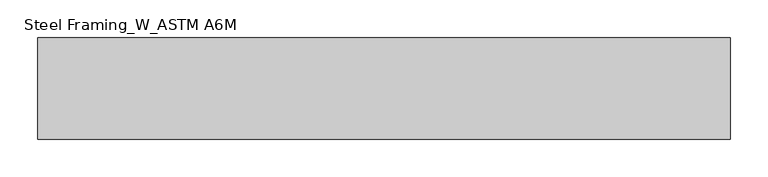
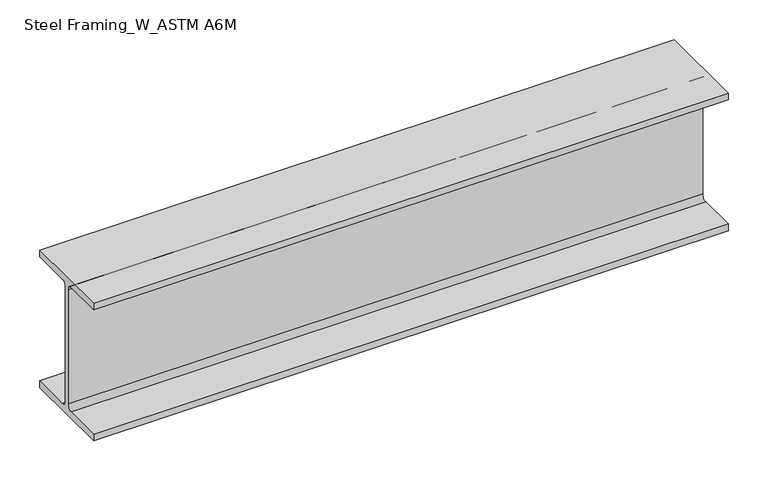
"""IFC4 building model written with IfcOpenShell, lengths in millimetres: beam geometry, Steel Framing_W_ASTM A6M : H_SB_AR_S02_W200x31.3_B6."""

import ifcopenshell
import ifcopenshell.guid

model = None  # the IFC model being written
_history = None  # IfcOwnerHistory: only IFC2X3 demands one
_inside = {}  # id of a spatial element -> (the spatial element, [elements in it])
_under = {}  # id of a project, library or spatial element -> (it, [spatial elements below it])
_declared = {}  # id of a project -> (the project, [libraries it declares])
_typed = {}  # id of a type object -> (the type object, [elements of that type])
_made_of = {}  # id of a material, layer set ... -> (it, [elements and type objects made of it])


def new_model(schema):
    """Start an empty IFC model of exactly this schema.

    Asked for "IFC4X3", IfcOpenShell would pick the latest addendum, in which some entities
    have other attributes; the version numbers below select the first issue.
    IFC2X3 requires an IfcOwnerHistory on every rooted entity: one is made here for all.
    """
    global model, _history
    if schema == "IFC4X3":
        model = ifcopenshell.file(schema_version=(4, 3, 0, 0))
    else:
        model = ifcopenshell.file(schema=schema)
    _inside.clear()
    _under.clear()
    _declared.clear()
    _typed.clear()
    _made_of.clear()
    _history = None
    if model.schema == "IFC2X3":
        org = make("IfcOrganization", Name="unknown")
        user = make(
            "IfcPersonAndOrganization",
            ThePerson=make("IfcPerson", FamilyName="unknown"),
            TheOrganization=org,
        )
        app = make(
            "IfcApplication",
            ApplicationDeveloper=org,
            Version="unknown",
            ApplicationFullName="unknown",
            ApplicationIdentifier="unknown",
        )
        _history = make(
            "IfcOwnerHistory",
            OwningUser=user,
            OwningApplication=app,
            ChangeAction="ADDED",
            CreationDate=0,
        )
    return model


def make(cls, **values):
    """One entity of the class cls with the attributes given. An attribute that is None is left unset."""
    return model.create_entity(
        cls, **{name: value for name, value in values.items() if value is not None}
    )


def rooted(cls, **values):
    """An entity with a GlobalId (a new one), such as an element, a storey or a relation."""
    return make(cls, GlobalId=ifcopenshell.guid.new(), OwnerHistory=_history, **values)


def si_unit(unit_type, name, prefix=None):
    """IfcSIUnit, for example si_unit("LENGTHUNIT", "METRE", prefix="MILLI")."""
    return make("IfcSIUnit", UnitType=unit_type, Prefix=prefix, Name=name)


def assignment(units):
    """IfcUnitAssignment: the units of a project."""
    return None if units is None else make("IfcUnitAssignment", Units=units)


def point(xyz):
    """IfcCartesianPoint."""
    return None if xyz is None else make("IfcCartesianPoint", Coordinates=xyz)


def direction(xyz):
    """IfcDirection."""
    return None if xyz is None else make("IfcDirection", DirectionRatios=xyz)


def frame(location, z_axis=None, x_axis=None):
    """IfcAxis2Placement3D, a coordinate frame: its origin and axes. An axis left out is left unset."""
    return make(
        "IfcAxis2Placement3D",
        Location=point(location),
        Axis=direction(z_axis),
        RefDirection=direction(x_axis),
    )


def frame_2d(location, x_axis=None):
    """IfcAxis2Placement2D, a coordinate frame in the plane: its origin and x axis."""
    return make(
        "IfcAxis2Placement2D", Location=point(location), RefDirection=direction(x_axis)
    )


def origin():
    """The frame at (0, 0, 0) with its axes left unset."""
    return frame((0.0, 0.0, 0.0))


def place(relative_to, where):
    """IfcLocalPlacement: puts the frame where relative to a parent placement (None: the world)."""
    return make(
        "IfcLocalPlacement", PlacementRelTo=relative_to, RelativePlacement=where
    )


def context(
    kind, dimensions, precision=None, world=None, true_north=None, identifier=None
):
    """IfcGeometricRepresentationContext, for example the 3D "Model" context."""
    return make(
        "IfcGeometricRepresentationContext",
        ContextIdentifier=identifier,
        ContextType=kind,
        CoordinateSpaceDimension=dimensions,
        Precision=precision,
        WorldCoordinateSystem=world,
        TrueNorth=true_north,
    )


def project(units=None, contexts=None):
    """IfcProject with its units and contexts."""
    return rooted(
        "IfcProject",
        Name="project",
        RepresentationContexts=contexts,
        UnitsInContext=assignment(units),
    )


def spatial(cls, under=None, at=None, **own):
    """A site, building, storey or space (cls), placed at a placement, below another one or the project."""
    s = rooted(cls, ObjectPlacement=at, **own)
    if under is not None:
        _under.setdefault(under.id(), (under, []))[1].append(s)
    return s


def polyline(points):
    """IfcPolyline through the points."""
    return make("IfcPolyline", Points=[point(p) for p in points])


def circle_curve(where, radius):
    """IfcCircle in the frame where."""
    return make("IfcCircle", Position=where, Radius=radius)


def trimmed(basis, trim1, trim2, sense, master):
    """IfcTrimmedCurve: the piece of a basis curve between two trims."""
    return make(
        "IfcTrimmedCurve",
        BasisCurve=basis,
        Trim1=trim1,
        Trim2=trim2,
        SenseAgreement=sense,
        MasterRepresentation=master,
    )


def segment(curve, same_sense, transition):
    """IfcCompositeCurveSegment."""
    return make(
        "IfcCompositeCurveSegment",
        Transition=transition,
        SameSense=same_sense,
        ParentCurve=curve,
    )


def composite_curve(segments, self_intersect=None):
    """IfcCompositeCurve: segments joined end to end."""
    return make("IfcCompositeCurve", Segments=segments, SelfIntersect=self_intersect)


def outline(outer, holes=None, kind="AREA"):
    """IfcArbitraryClosedProfileDef: a profile drawn as a closed curve; with holes, ...WithVoids."""
    if holes is None:
        return make("IfcArbitraryClosedProfileDef", ProfileType=kind, OuterCurve=outer)
    return make(
        "IfcArbitraryProfileDefWithVoids",
        ProfileType=kind,
        OuterCurve=outer,
        InnerCurves=holes,
    )


def extrude(swept, where, along, depth):
    """IfcExtrudedAreaSolid: the profile swept, set in the frame where, extruded along a direction by depth."""
    return make(
        "IfcExtrudedAreaSolid",
        SweptArea=swept,
        Position=where,
        ExtrudedDirection=direction(along),
        Depth=depth,
    )


def shape(context_of_items, identifier, shape_type, items):
    """IfcShapeRepresentation: the items that make up one representation, for example the "Body"."""
    return make(
        "IfcShapeRepresentation",
        ContextOfItems=context_of_items,
        RepresentationIdentifier=identifier,
        RepresentationType=shape_type,
        Items=items,
    )


def source(mapping_origin, context_of_items, identifier, shape_type, items):
    """IfcRepresentationMap: a shape defined once, which mapped items show again and again."""
    return make(
        "IfcRepresentationMap",
        MappingOrigin=mapping_origin,
        MappedRepresentation=shape(context_of_items, identifier, shape_type, items),
    )


def transform(
    local_origin,
    x_axis=None,
    y_axis=None,
    z_axis=None,
    scale=None,
    scale2=None,
    scale3=None,
    uniform=True,
):
    """IfcCartesianTransformationOperator3D, or its non-uniform kind. x_axis, y_axis, z_axis: its Axis1, 2, 3."""
    if uniform:
        return make(
            "IfcCartesianTransformationOperator3D",
            Axis1=direction(x_axis),
            Axis2=direction(y_axis),
            LocalOrigin=point(local_origin),
            Scale=scale,
            Axis3=direction(z_axis),
        )
    return make(
        "IfcCartesianTransformationOperator3DnonUniform",
        Axis1=direction(x_axis),
        Axis2=direction(y_axis),
        LocalOrigin=point(local_origin),
        Scale=scale,
        Axis3=direction(z_axis),
        Scale2=scale2,
        Scale3=scale3,
    )


def mapped(mapping_source, mapping_target):
    """IfcMappedItem: shows the shape of a source again, moved by a transform."""
    return make(
        "IfcMappedItem", MappingSource=mapping_source, MappingTarget=mapping_target
    )


def made_of(thing, what):
    """Note that an element or type object is made of a material, layer set ...; save() writes the relation."""
    if what is not None:
        _made_of.setdefault(what.id(), (what, []))[1].append(thing)
    return thing


def element(
    cls,
    number,
    at=None,
    inside=None,
    cuts=None,
    type_object=None,
    material=None,
    context=None,
    identifier="Body",
    shape_type=None,
    held_by="IfcProductDefinitionShape",
    body=None,
    shapes=None,
    **own,
):
    """One element of the class cls, such as IfcWall. Its Tag is "e" and its number.

    at: its placement. inside: the storey or other place that contains it. cuts: it is an
    opening in that element (IfcRelVoidsElement). A single representation is given by context,
    identifier, shape_type and body (its items); several are given by shapes. held_by: the class
    of the entity that holds the representations. save() writes the other relations.
    """
    e = rooted(cls, Tag="e%d" % number, ObjectPlacement=at, **own)
    if body is not None:
        shapes = [shape(context, identifier, shape_type, body)]
    if shapes is not None:
        e.Representation = make(held_by, Representations=shapes)
    if inside is not None:
        _inside.setdefault(inside.id(), (inside, []))[1].append(e)
    if cuts is not None:
        rooted(
            "IfcRelVoidsElement", RelatingBuildingElement=cuts, RelatedOpeningElement=e
        )
    if type_object is not None:
        _typed.setdefault(type_object.id(), (type_object, []))[1].append(e)
    return made_of(e, material)


def aggregate(whole, parts):
    """IfcRelAggregates: a whole, such as a stair, and the parts it consists of."""
    return rooted("IfcRelAggregates", RelatingObject=whole, RelatedObjects=parts)


def save(model, path):
    """Write the relations noted so far, then the file.

    IfcRelAggregates (storeys below a building ...), IfcRelContainedInSpatialStructure (elements
    in a storey), IfcRelDefinesByType, IfcRelAssociatesMaterial and IfcRelDeclares: one each for
    every whole, place, type object, material and project.
    """
    for whole, parts in _under.values():
        aggregate(whole, parts)
    for where, things in _inside.values():
        rooted(
            "IfcRelContainedInSpatialStructure",
            RelatedElements=things,
            RelatingStructure=where,
        )
    for kind, things in _typed.values():
        rooted("IfcRelDefinesByType", RelatedObjects=things, RelatingType=kind)
    for what, things in _made_of.values():
        rooted("IfcRelAssociatesMaterial", RelatedObjects=things, RelatingMaterial=what)
    for by, libraries in _declared.values():
        rooted("IfcRelDeclares", RelatingContext=by, RelatedDefinitions=libraries)
    model.write(path)


def steel_framing_w_astm_a6m_90a0bae4(model_context):
    return source(origin(), model_context, "Body", "SweptSolid", [
        extrude(outline(composite_curve([segment(polyline([(67.0, -94.8), (67.0, -105.0), (-67.0, -105.0), (-67.0, -94.8), (-10.775, -94.8)]), True, "CONTINUOUS"), segment(trimmed(circle_curve(frame_2d((-10.775, -87.2)), 7.6), [point((-10.775, -94.8))], [point((-3.175, -87.2))], True, "CARTESIAN"), True, "CONTINUOUS"), segment(polyline([(-3.175, -87.2), (-3.175, 87.2)]), True, "CONTINUOUS"), segment(trimmed(circle_curve(frame_2d((-10.775, 87.2)), 7.6), [point((-3.175, 87.2))], [point((-10.775, 94.8))], True, "CARTESIAN"), True, "CONTINUOUS"), segment(polyline([(-10.775, 94.8), (-67.0, 94.8), (-67.0, 105.0), (67.0, 105.0), (67.0, 94.8), (10.775, 94.8)]), True, "CONTINUOUS"), segment(trimmed(circle_curve(frame_2d((10.775, 87.2)), 7.6), [point((10.775, 94.8))], [point((3.175, 87.2))], True, "CARTESIAN"), True, "CONTINUOUS"), segment(polyline([(3.175, 87.2), (3.175, -87.2)]), True, "CONTINUOUS"), segment(trimmed(circle_curve(frame_2d((10.775, -87.2)), 7.6), [point((3.175, -87.2))], [point((10.775, -94.8))], True, "CARTESIAN"), True, "CONTINUOUS"), segment(polyline([(10.775, -94.8), (67.0, -94.8)]), True, "CONTINUOUS")], self_intersect=False)), frame((-421.3, 0.0, 0.0), z_axis=(1.0, 0.0, 0.0), x_axis=(0.0, 1.0, 0.0)), (0.0, 0.0, 1.0), 916.6),
    ])


if __name__ == "__main__":
    model = new_model("IFC4")
    model_context = context("Model", 3, world=origin())
    ifc_project = project(units=[si_unit("LENGTHUNIT", "METRE", prefix="MILLI")], contexts=[model_context])
    site = spatial("IfcSite", under=ifc_project)
    building = spatial("IfcBuilding", under=site)
    placement = place(None, origin())
    steel_framing_w_astm_a6m_shape = steel_framing_w_astm_a6m_90a0bae4(model_context)
    element("IfcBeam", 1, ObjectType="Steel Framing_W_ASTM A6M : H_SB_AR_S02_W200x31.3_B6", at=placement, inside=building, context=model_context, shape_type="MappedRepresentation", body=[
        mapped(steel_framing_w_astm_a6m_shape, transform((0.0, 0.0, 0.0), x_axis=(1.0, 0.0, 0.0), y_axis=(0.0, 1.0, 0.0), z_axis=(0.0, 0.0, 1.0))),
    ])
    save(model, "model.ifc")

# Revit data of these elements
# Type "Steel Framing_W_ASTM A6M : H_SB_AR_S02_W200x31.3_B6"
#   Type Mark = "B6"
#   Section Name Key = "W8x21"
#   Width = 13.4 cm
#   Web Thickness = 0.635 cm
#   Web Fillet = 0.76 cm
#   Warping Constant = 40800.0 cm⁶
#   Torsional Moment of Inertia = 11.70 cm⁴
#   Section Area = 39.7 cm²
#   Plastic Modulus weak axis = 93.2 cm³
#   Plastic Modulus strong axis = 334.0 cm³
#   Perimeter = 0.93 m²/m
#   Nominal Weight = 31.30 kgf/m
#   Moment of Inertia weak axis = 407.00 cm⁴
#   Moment of Inertia strong axis = 3130.00 cm⁴
#   Height = 21.0 cm
#   Flange Thickness = 1.02 cm
#   Elastic Modulus weak axis = 60.8 cm³
#   Elastic Modulus strong axis = 298.0 cm³
#   Centroid Vertical = 10.5 cm
#   Centroid Horizontal = 6.7 cm
#   Length [instance default] = 1500 mm
#   Structural Material [instance default] = Steel, 45-345
#   Bolt Spacing = 0
#   Assembly Code = ""
# Element 1 (IfcBeam, "Steel Framing_W_ASTM A6M : H_SB_AR_S02_W200x31.3_B6")
#   Materials on its faces: "Steel, 45-345"
# Materials
#   "Steel, 45-345": class "Metal", colour RGB 189 187 185, transparency 0, Description = "Steel 345 MPa", Cost = 0
